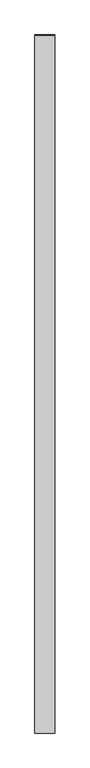
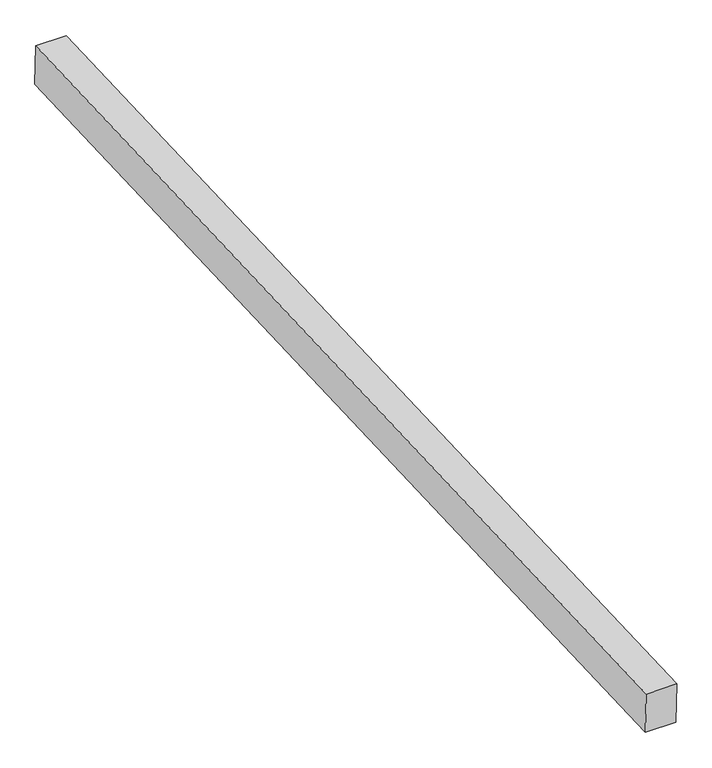
"""IFC4 building model written with IfcOpenShell, lengths in millimetres: proxy geometry, Generic Models 7:Generic Models 1:8:Generic Models 1:8 : Generic Models 7:Generic Models 1:337419:27 : Generic Models 7:Generic Models 1:8:Generic Models 1:8 : Generic Models 7:Generic Models 1:337419:315935."""

from ifc_helpers import new_model, si_unit, frame, origin, place, context, project, spatial, polyline, outline, extrude, source, transform, mapped, element, save


def generic_models_faac03d7(model_context):
    return source(origin(), model_context, "Body", "SweptSolid", [
        extrude(outline(polyline([(-569809.5331551, 8697.9424054), (-564936.6102609, 8900.9808594), (-564929.0433392, 8710.6308549), (-569801.6025364, 8507.607555), (-569809.5331551, 8697.9424054)])), frame((591213.9617243, 0.0, 0.0), z_axis=(1.0, 0.0, 0.0), x_axis=(0.0, 1.0, 0.0)), (0.0, 0.0, 1.0), 139.7),
    ])


if __name__ == "__main__":
    model = new_model("IFC4")
    model_context = context("Model", 3, world=origin())
    ifc_project = project(units=[si_unit("LENGTHUNIT", "METRE", prefix="MILLI")], contexts=[model_context])
    site = spatial("IfcSite", under=ifc_project)
    building = spatial("IfcBuilding", under=site)
    placement = place(None, origin())
    generic_models_shape = generic_models_faac03d7(model_context)
    element("IfcBuildingElementProxy", 1, Name="Generic Models 7:Generic Models 1:8:Generic Models 1:8 : Generic Models 7:Generic Models 1:337419:27 : Generic Models 7:Generic Models 1:8:Generic Models 1:8 : Generic Models 7:Generic Models 1:337419:315935", ObjectType="Generic Models 7:Generic Models 1:8:Generic Models 1:8 : Generic Models 7:Generic Models 1:337419:27 : Generic Models 7:Generic Models 1:8:Generic Models 1:8 : Generic Models 7:Generic Models 1:337419:315935", at=placement, inside=building, context=model_context, shape_type="MappedRepresentation", body=[
        mapped(generic_models_shape, transform((0.0, 0.0, 0.0), x_axis=(1.0, 0.0, 0.0), y_axis=(0.0, 1.0, 0.0), z_axis=(0.0, 0.0, 1.0))),
    ])
    save(model, "model.ifc")

# Revit data of these elements
# Type "Generic Models 7:Generic Models 1:8:Generic Models 1:8 : Generic Models 7:Generic Models 1:337419:27 : Generic Models 7:Generic Models 1:8:Generic Models 1:8 : Generic Models 7:Generic Models 1:337419:315935"
#   NameOverride = "Generic Models 7:Generic Models 1:8:Generic Models 1:8 : Generic Models 7:Generic Models 1:337419:315935"
#   ObjectTypeOverride = "Generic Models 1:8 : Generic Models 7:Generic Models 1:337419"
#   Reference = "Generic Models 1"
#   Tag = "315935"
# Element 1 (IfcBuildingElementProxy, "Generic Models 7:Generic Models 1:8:Generic Models 1:8 : Generic Models 7:Generic Models 1:337419:27 : Generic Models 7:Generic Models 1:8:Generic Models 1:8 : Generic Models 7:Generic Models 1:337419:315935")
#   Materials on its faces: "5 1/2\" X 7 1/2\" EXTERIOR GRADE GLULAM BEAMS"
# Materials
#   "5 1/2\" X 7 1/2\" EXTERIOR GRADE GLULAM BEAMS": class "Wood", colour RGB 183 134 68, transparency 0, Keynote = "M06181300.01", Description = "Pinus Echinata", Cost = 0
